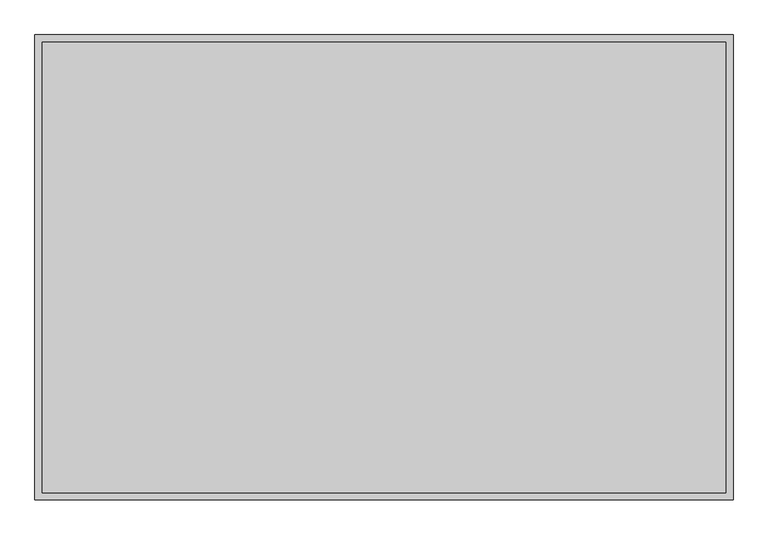
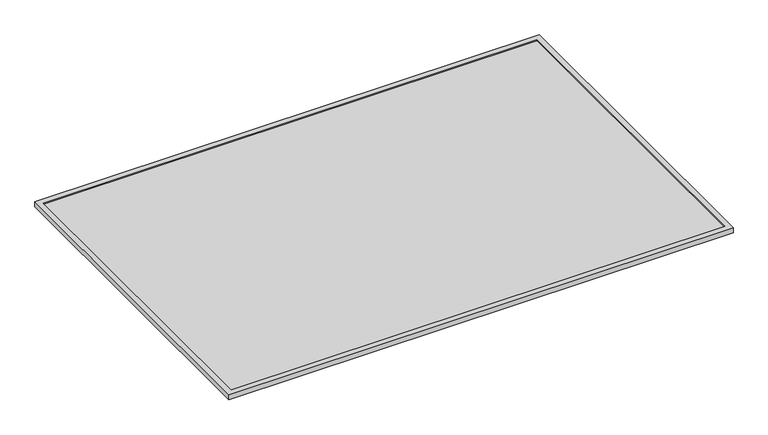
"""IFC4 building model written with IfcOpenShell, lengths in millimetres: proxy geometry, Bradley-Washroom_Accessories-Mirrors-780_Custom : Bradley-Washroom_Accessories-Mirrors-780_Custom."""

from ifc_helpers import new_model, si_unit, frame, origin, place, context, project, spatial, polyline, outline, extrude, faceted_brep, source, transform, mapped, element, save


def specialty_equipment_0bafb7ae(model_context):
    return source(origin(), model_context, "Body", "SolidModel", [
        extrude(outline(polyline([(895.35, 590.55), (895.35, -590.55), (-895.35, -590.55), (-895.35, 590.55), (895.35, 590.55)])), frame((0.0, 0.0, 9.525), z_axis=(0.0, 0.0, 1.0), x_axis=(1.0, 0.0, 0.0)), (0.0, 0.0, 1.0), 4.7625),
        faceted_brep([(914.4, 609.6, 19.05), (-914.4, 609.6, 19.05), (-914.4, -609.6, 19.05), (914.4, -609.6, 19.05), (-895.35, 590.55, 19.05), (895.35, 590.55, 19.05), (895.35, -590.55, 19.05), (-895.35, -590.55, 19.05), (914.4, 609.6, 0.0), (914.4, -609.6, 0.0), (-914.4, -609.6, 0.0), (-914.4, 609.6, 0.0), (895.35, 590.55, 9.525), (-895.35, 590.55, 9.525), (-895.35, -590.55, 9.525), (895.35, -590.55, 9.525)], [[[0, 1, 2, 3], [4, 5, 6, 7]], [[8, 9, 10, 11]], [[1, 0, 8, 11]], [[2, 1, 11, 10]], [[3, 2, 10, 9]], [[0, 3, 9, 8]], [[12, 13, 14, 15]], [[13, 12, 5, 4]], [[14, 13, 4, 7]], [[15, 14, 7, 6]], [[12, 15, 6, 5]]]),
    ])


if __name__ == "__main__":
    model = new_model("IFC4")
    model_context = context("Model", 3, world=origin())
    ifc_project = project(units=[si_unit("LENGTHUNIT", "METRE", prefix="MILLI")], contexts=[model_context])
    site = spatial("IfcSite", under=ifc_project)
    building = spatial("IfcBuilding", under=site)
    placement = place(None, origin())
    specialty_equipment_shape = specialty_equipment_0bafb7ae(model_context)
    element("IfcBuildingElementProxy", 1, Name="Bradley-Washroom_Accessories-Mirrors-780_Custom : Bradley-Washroom_Accessories-Mirrors-780_Custom", ObjectType="Bradley-Washroom_Accessories-Mirrors-780_Custom : Bradley-Washroom_Accessories-Mirrors-780_Custom", at=placement, inside=building, context=model_context, shape_type="MappedRepresentation", body=[
        mapped(specialty_equipment_shape, transform((0.0, 0.0, 0.0), x_axis=(1.0, 0.0, 0.0), y_axis=(0.0, 1.0, 0.0), z_axis=(0.0, 0.0, 1.0))),
    ])
    save(model, "model.ifc")

# Revit data of these elements
# Type "Bradley-Washroom_Accessories-Mirrors-780_Custom : Bradley-Washroom_Accessories-Mirrors-780_Custom"
#   Warranty Information = "Complete unit, excepting mirrors warranted for one year.\r\n Stainless steel mirror frames for fifteen years.\r\n Plate glass mirrors for fifteen years.\r\n This warranty does not cover installation or any other labor charges and does not apply to any units,\r\n which have been damaged by accident, abuse, improper installation, improper maintenance, or altered in any way."
#   Version = "1.0"
#   URL = "http://www.bradleycorp.com/"
#   Type Comments = "ERROR - If you are able to see this message you haven't loaded this  family correctly."
#   OmniClass Title = "Mirrors"
#   OmniClass Code = "23.40.95.17.17"
#   Modeling Code = ""
#   Model = "ERROR - If you are able to see this message you haven't loaded this  family correctly."
#   MasterFormat Title = "Commercial Toilet Accessories"
#   MasterFormat Number = "10 28 13. 13"
#   Manufacturer = "Bradley Corporation"
#   Keynote = "M08831300.01"
#   Industry Standards = "ASTM C 1036"
#   Fire Rating = "n/a"
#   Dimensional Limits [instance default] = "Either Width or Hight must be over 25\""
#   Description = "ERROR - If you are able to see this message you haven't loaded this  family correctly."
#   Copyright = "This Model Data is Property of Bradley Corporation"
#   Buy American Act = "Yes"
#   Assembly Code = "C1030900"
#   ADA Compliant = "Yes"
#   Width [instance default] = 1' - 6"
#   Total Width [instance default] = 1' - 6"
#   Total Height [instance default] = 3' - 0"
#   Height [instance default] = 3' - 0"
#   Depth [instance default] = 0' - 0 3/4"
#   Default Elevation = 3' - 4"
#   Reflective Material = Glass - Bradley Corp - BradEX - Polished Float Mirror
#   Frame Material = Bradley Corp Stainless Steel - Satin
# Element 1 (IfcBuildingElementProxy, "Bradley-Washroom_Accessories-Mirrors-780_Custom : Bradley-Washroom_Accessories-Mirrors-780_Custom")
#   Width = 6' - 0"
#   Total Width = 6' - 0"
#   Total Height = 4' - 0"
#   Height = 4' - 0"
#   Materials on its faces: "Bradley Corp Stainless Steel - Satin", "Glass - Bradley Corp - BradEX - Polished Float Mirror"
# Materials
#   "Glass - Bradley Corp - BradEX - Polished Float Mirror": class "Glass", colour RGB 221 230 232, transparency 0, Manufacturer = "Bradley Corporation", URL = "www.bradleycorp.com", Description = "Stainless Steel - Satin Finish", Cost = 0
#   "Bradley Corp Stainless Steel - Satin": class "Metal", colour RGB 189 187 185, transparency 0, Manufacturer = "Bradley Corporation", URL = "www.bradleycorp.com", Description = "Stainless Steel - Satin Finish", Cost = 0
